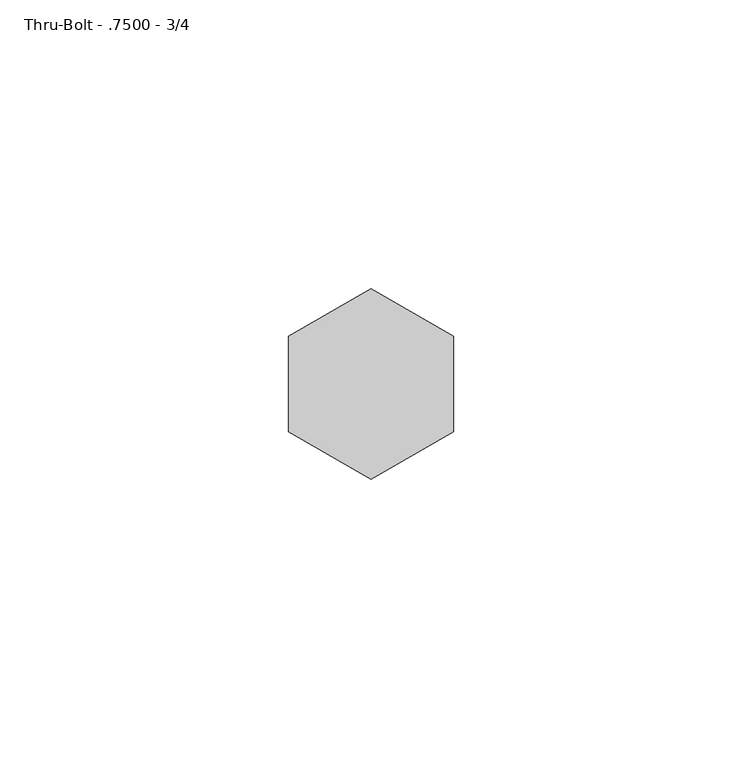
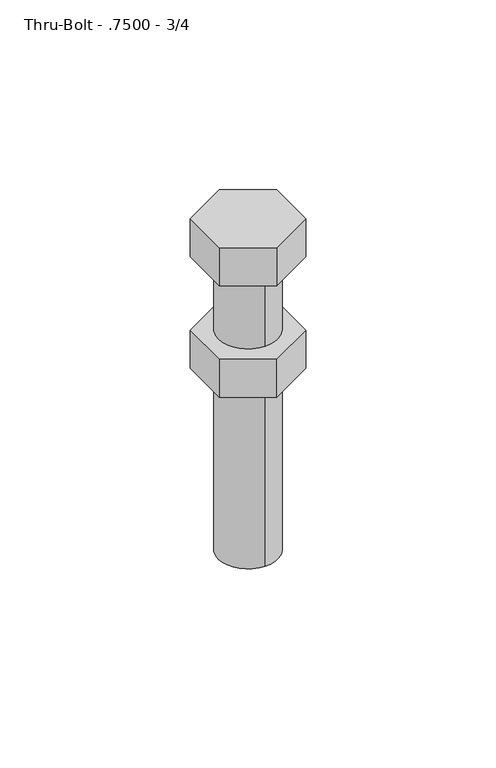
"""IFC4 building model written with IfcOpenShell, lengths in millimetres: fastener geometry, 060523 - W_P_C - Fastenings - Generic : Thru-Bolt - .7500 - 3/4."""

from ifc_helpers import new_model, si_unit, point, frame, origin, origin_with_axes, origin_2d, place, context, project, spatial, polyline, circle_curve, trimmed, segment, composite_curve, outline, extrude, source, transform, mapped, element, save


def thru_bolt_7500_3_4_06f79f2f(model_context):
    return source(origin(), model_context, "Body", "SweptSolid", [
        extrude(outline(polyline([(-14.2875, -8.248892), (-14.2875, 8.248892), (0.0, 16.4977839), (14.2875, 8.248892), (14.2875, -8.248892), (0.0, -16.4977839), (-14.2875, -8.248892)])), frame((0.0, 0.0, -38.6953125), z_axis=(0.0, 0.0, 1.0), x_axis=(1.0, 0.0, 0.0)), (0.0, 0.0, 1.0), 13.2953125),
        extrude(outline(polyline([(-14.2875, 8.248892), (0.0, 16.4977839), (14.2875, 8.248892), (14.2875, -8.248892), (0.0, -16.4977839), (-14.2875, -8.248892), (-14.2875, 8.248892)])), origin_with_axes(), (0.0, 0.0, 1.0), 13.2953125),
        extrude(outline(composite_curve([segment(trimmed(circle_curve(origin_2d(), 9.7730469), [point((0.0, -9.7730469))], [point((0.0, 9.7730469))], False, "CARTESIAN"), True, "CONTINUOUS"), segment(trimmed(circle_curve(origin_2d(), 9.7730469), [point((0.0, 9.7730469))], [point((0.0, -9.7730469))], False, "CARTESIAN"), True, "CONTINUOUS")], self_intersect=False)), frame((0.0, 0.0, -101.6), z_axis=(0.0, 0.0, 1.0), x_axis=(1.0, 0.0, 0.0)), (0.0, 0.0, 1.0), 101.6),
    ])


if __name__ == "__main__":
    model = new_model("IFC4")
    model_context = context("Model", 3, world=origin())
    ifc_project = project(units=[si_unit("LENGTHUNIT", "METRE", prefix="MILLI")], contexts=[model_context])
    site = spatial("IfcSite", under=ifc_project)
    building = spatial("IfcBuilding", under=site)
    placement = place(None, origin())
    thru_bolt_7500_3_4_shape = thru_bolt_7500_3_4_06f79f2f(model_context)
    element("IfcFastener", 1, ObjectType="060523 - W_P_C - Fastenings - Generic : Thru-Bolt - .7500 - 3/4", at=placement, inside=building, context=model_context, shape_type="MappedRepresentation", body=[
        mapped(thru_bolt_7500_3_4_shape, transform((0.0, 0.0, 0.0), x_axis=(1.0, 0.0, 0.0), y_axis=(0.0, 1.0, 0.0), z_axis=(0.0, 0.0, 1.0))),
    ])
    save(model, "model.ifc")

# Revit data of these elements
# Type "060523 - W_P_C - Fastenings - Generic : Thru-Bolt - .7500 - 3/4"
#   Washer_Thickness = 0' - 0.17448"
#   Washer Radius = 0' - 0.9082"
#   Washer Offset - Head = 0' - 0"
#   Washer Offset = 0' - 0"
#   Thickness_of_Substrate [instance default] = 0' - 1"
#   Side = 0' - 0.65039"
#   Radius = 0' - 0.38477"
#   Length [instance default] = 0' - 4"
#   Head Size = 0' - 1 1/8"
#   Head Radius = 0' - 0 9/16"
#   Head Height = 0' - 0 67/128"
#   Double Diameter = 0' - 1 69/128"
#   Diameter = 0' - 0 197/256"
#   Default Elevation = 4' - 0"
#   Washer_Nut_Visibility = no
#   Washer_Head_Visibility = no
#   Round_Head_Visibility = no
#   Point Visibility = no
#   Nut_Visibility = yes
#   Hex_Head_Visiblilty = yes
#   Washer Material = none
#   Bolt Material (Size) = AT SILL - FASTENER AT 24" O.C.
# Element 1 (IfcFastener, "060523 - W_P_C - Fastenings - Generic : Thru-Bolt - .7500 - 3/4")
#   Materials on its faces: "AT SILL - FASTENER AT 24\" O.C."
# Materials
#   "AT SILL - FASTENER AT 24\" O.C.": class "Generic", colour RGB 120 120 120, transparency 0, Cost = 0
